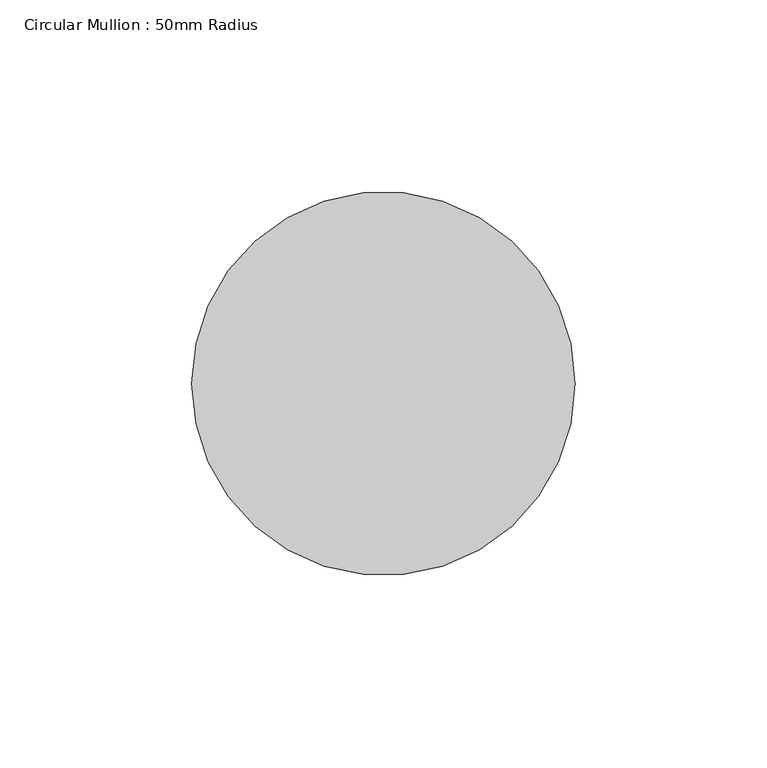
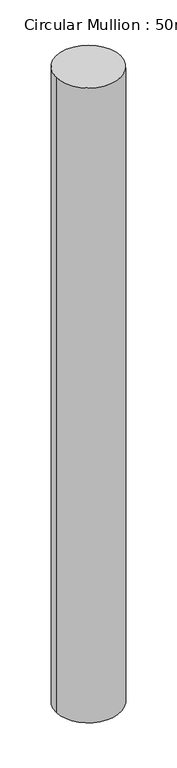
"""IFC4 building model written with IfcOpenShell, lengths in millimetres: member geometry, Circular Mullion : 50mm Radius."""

import ifcopenshell
import ifcopenshell.guid

model = None  # the IFC model being written
_history = None  # IfcOwnerHistory: only IFC2X3 demands one
_inside = {}  # id of a spatial element -> (the spatial element, [elements in it])
_under = {}  # id of a project, library or spatial element -> (it, [spatial elements below it])
_declared = {}  # id of a project -> (the project, [libraries it declares])
_typed = {}  # id of a type object -> (the type object, [elements of that type])
_made_of = {}  # id of a material, layer set ... -> (it, [elements and type objects made of it])


def new_model(schema):
    """Start an empty IFC model of exactly this schema.

    Asked for "IFC4X3", IfcOpenShell would pick the latest addendum, in which some entities
    have other attributes; the version numbers below select the first issue.
    IFC2X3 requires an IfcOwnerHistory on every rooted entity: one is made here for all.
    """
    global model, _history
    if schema == "IFC4X3":
        model = ifcopenshell.file(schema_version=(4, 3, 0, 0))
    else:
        model = ifcopenshell.file(schema=schema)
    _inside.clear()
    _under.clear()
    _declared.clear()
    _typed.clear()
    _made_of.clear()
    _history = None
    if model.schema == "IFC2X3":
        org = make("IfcOrganization", Name="unknown")
        user = make(
            "IfcPersonAndOrganization",
            ThePerson=make("IfcPerson", FamilyName="unknown"),
            TheOrganization=org,
        )
        app = make(
            "IfcApplication",
            ApplicationDeveloper=org,
            Version="unknown",
            ApplicationFullName="unknown",
            ApplicationIdentifier="unknown",
        )
        _history = make(
            "IfcOwnerHistory",
            OwningUser=user,
            OwningApplication=app,
            ChangeAction="ADDED",
            CreationDate=0,
        )
    return model


def make(cls, **values):
    """One entity of the class cls with the attributes given. An attribute that is None is left unset."""
    return model.create_entity(
        cls, **{name: value for name, value in values.items() if value is not None}
    )


def rooted(cls, **values):
    """An entity with a GlobalId (a new one), such as an element, a storey or a relation."""
    return make(cls, GlobalId=ifcopenshell.guid.new(), OwnerHistory=_history, **values)


def si_unit(unit_type, name, prefix=None):
    """IfcSIUnit, for example si_unit("LENGTHUNIT", "METRE", prefix="MILLI")."""
    return make("IfcSIUnit", UnitType=unit_type, Prefix=prefix, Name=name)


def assignment(units):
    """IfcUnitAssignment: the units of a project."""
    return None if units is None else make("IfcUnitAssignment", Units=units)


def point(xyz):
    """IfcCartesianPoint."""
    return None if xyz is None else make("IfcCartesianPoint", Coordinates=xyz)


def direction(xyz):
    """IfcDirection."""
    return None if xyz is None else make("IfcDirection", DirectionRatios=xyz)


def frame(location, z_axis=None, x_axis=None):
    """IfcAxis2Placement3D, a coordinate frame: its origin and axes. An axis left out is left unset."""
    return make(
        "IfcAxis2Placement3D",
        Location=point(location),
        Axis=direction(z_axis),
        RefDirection=direction(x_axis),
    )


def frame_2d(location, x_axis=None):
    """IfcAxis2Placement2D, a coordinate frame in the plane: its origin and x axis."""
    return make(
        "IfcAxis2Placement2D", Location=point(location), RefDirection=direction(x_axis)
    )


def origin():
    """The frame at (0, 0, 0) with its axes left unset."""
    return frame((0.0, 0.0, 0.0))


def origin_2d():
    """The frame at (0, 0) in the plane with its x axis left unset."""
    return frame_2d((0.0, 0.0))


def place(relative_to, where):
    """IfcLocalPlacement: puts the frame where relative to a parent placement (None: the world)."""
    return make(
        "IfcLocalPlacement", PlacementRelTo=relative_to, RelativePlacement=where
    )


def context(
    kind, dimensions, precision=None, world=None, true_north=None, identifier=None
):
    """IfcGeometricRepresentationContext, for example the 3D "Model" context."""
    return make(
        "IfcGeometricRepresentationContext",
        ContextIdentifier=identifier,
        ContextType=kind,
        CoordinateSpaceDimension=dimensions,
        Precision=precision,
        WorldCoordinateSystem=world,
        TrueNorth=true_north,
    )


def project(units=None, contexts=None):
    """IfcProject with its units and contexts."""
    return rooted(
        "IfcProject",
        Name="project",
        RepresentationContexts=contexts,
        UnitsInContext=assignment(units),
    )


def spatial(cls, under=None, at=None, **own):
    """A site, building, storey or space (cls), placed at a placement, below another one or the project."""
    s = rooted(cls, ObjectPlacement=at, **own)
    if under is not None:
        _under.setdefault(under.id(), (under, []))[1].append(s)
    return s


def circle_curve(where, radius):
    """IfcCircle in the frame where."""
    return make("IfcCircle", Position=where, Radius=radius)


def trimmed(basis, trim1, trim2, sense, master):
    """IfcTrimmedCurve: the piece of a basis curve between two trims."""
    return make(
        "IfcTrimmedCurve",
        BasisCurve=basis,
        Trim1=trim1,
        Trim2=trim2,
        SenseAgreement=sense,
        MasterRepresentation=master,
    )


def segment(curve, same_sense, transition):
    """IfcCompositeCurveSegment."""
    return make(
        "IfcCompositeCurveSegment",
        Transition=transition,
        SameSense=same_sense,
        ParentCurve=curve,
    )


def composite_curve(segments, self_intersect=None):
    """IfcCompositeCurve: segments joined end to end."""
    return make("IfcCompositeCurve", Segments=segments, SelfIntersect=self_intersect)


def outline(outer, holes=None, kind="AREA"):
    """IfcArbitraryClosedProfileDef: a profile drawn as a closed curve; with holes, ...WithVoids."""
    if holes is None:
        return make("IfcArbitraryClosedProfileDef", ProfileType=kind, OuterCurve=outer)
    return make(
        "IfcArbitraryProfileDefWithVoids",
        ProfileType=kind,
        OuterCurve=outer,
        InnerCurves=holes,
    )


def extrude(swept, where, along, depth):
    """IfcExtrudedAreaSolid: the profile swept, set in the frame where, extruded along a direction by depth."""
    return make(
        "IfcExtrudedAreaSolid",
        SweptArea=swept,
        Position=where,
        ExtrudedDirection=direction(along),
        Depth=depth,
    )


def shape(context_of_items, identifier, shape_type, items):
    """IfcShapeRepresentation: the items that make up one representation, for example the "Body"."""
    return make(
        "IfcShapeRepresentation",
        ContextOfItems=context_of_items,
        RepresentationIdentifier=identifier,
        RepresentationType=shape_type,
        Items=items,
    )


def source(mapping_origin, context_of_items, identifier, shape_type, items):
    """IfcRepresentationMap: a shape defined once, which mapped items show again and again."""
    return make(
        "IfcRepresentationMap",
        MappingOrigin=mapping_origin,
        MappedRepresentation=shape(context_of_items, identifier, shape_type, items),
    )


def transform(
    local_origin,
    x_axis=None,
    y_axis=None,
    z_axis=None,
    scale=None,
    scale2=None,
    scale3=None,
    uniform=True,
):
    """IfcCartesianTransformationOperator3D, or its non-uniform kind. x_axis, y_axis, z_axis: its Axis1, 2, 3."""
    if uniform:
        return make(
            "IfcCartesianTransformationOperator3D",
            Axis1=direction(x_axis),
            Axis2=direction(y_axis),
            LocalOrigin=point(local_origin),
            Scale=scale,
            Axis3=direction(z_axis),
        )
    return make(
        "IfcCartesianTransformationOperator3DnonUniform",
        Axis1=direction(x_axis),
        Axis2=direction(y_axis),
        LocalOrigin=point(local_origin),
        Scale=scale,
        Axis3=direction(z_axis),
        Scale2=scale2,
        Scale3=scale3,
    )


def mapped(mapping_source, mapping_target):
    """IfcMappedItem: shows the shape of a source again, moved by a transform."""
    return make(
        "IfcMappedItem", MappingSource=mapping_source, MappingTarget=mapping_target
    )


def made_of(thing, what):
    """Note that an element or type object is made of a material, layer set ...; save() writes the relation."""
    if what is not None:
        _made_of.setdefault(what.id(), (what, []))[1].append(thing)
    return thing


def element(
    cls,
    number,
    at=None,
    inside=None,
    cuts=None,
    type_object=None,
    material=None,
    context=None,
    identifier="Body",
    shape_type=None,
    held_by="IfcProductDefinitionShape",
    body=None,
    shapes=None,
    **own,
):
    """One element of the class cls, such as IfcWall. Its Tag is "e" and its number.

    at: its placement. inside: the storey or other place that contains it. cuts: it is an
    opening in that element (IfcRelVoidsElement). A single representation is given by context,
    identifier, shape_type and body (its items); several are given by shapes. held_by: the class
    of the entity that holds the representations. save() writes the other relations.
    """
    e = rooted(cls, Tag="e%d" % number, ObjectPlacement=at, **own)
    if body is not None:
        shapes = [shape(context, identifier, shape_type, body)]
    if shapes is not None:
        e.Representation = make(held_by, Representations=shapes)
    if inside is not None:
        _inside.setdefault(inside.id(), (inside, []))[1].append(e)
    if cuts is not None:
        rooted(
            "IfcRelVoidsElement", RelatingBuildingElement=cuts, RelatedOpeningElement=e
        )
    if type_object is not None:
        _typed.setdefault(type_object.id(), (type_object, []))[1].append(e)
    return made_of(e, material)


def aggregate(whole, parts):
    """IfcRelAggregates: a whole, such as a stair, and the parts it consists of."""
    return rooted("IfcRelAggregates", RelatingObject=whole, RelatedObjects=parts)


def save(model, path):
    """Write the relations noted so far, then the file.

    IfcRelAggregates (storeys below a building ...), IfcRelContainedInSpatialStructure (elements
    in a storey), IfcRelDefinesByType, IfcRelAssociatesMaterial and IfcRelDeclares: one each for
    every whole, place, type object, material and project.
    """
    for whole, parts in _under.values():
        aggregate(whole, parts)
    for where, things in _inside.values():
        rooted(
            "IfcRelContainedInSpatialStructure",
            RelatedElements=things,
            RelatingStructure=where,
        )
    for kind, things in _typed.values():
        rooted("IfcRelDefinesByType", RelatedObjects=things, RelatingType=kind)
    for what, things in _made_of.values():
        rooted("IfcRelAssociatesMaterial", RelatedObjects=things, RelatingMaterial=what)
    for by, libraries in _declared.values():
        rooted("IfcRelDeclares", RelatingContext=by, RelatedDefinitions=libraries)
    model.write(path)


def circular_mullion_50mm_radius_d9d2f8d6(model_context):
    return source(origin(), model_context, "Body", "SweptSolid", [
        extrude(outline(composite_curve([segment(trimmed(circle_curve(origin_2d(), 50.0), [point((50.0, 0.0))], [point((-50.0, 0.0))], False, "CARTESIAN"), True, "CONTINUOUS"), segment(trimmed(circle_curve(origin_2d(), 50.0), [point((-50.0, 0.0))], [point((50.0, 0.0))], False, "CARTESIAN"), True, "CONTINUOUS")], self_intersect=False)), frame((0.0, 0.0, -1037.8609437), z_axis=(0.0, 0.0, 1.0), x_axis=(1.0, 0.0, 0.0)), (0.0, 0.0, 1.0), 1037.8609437),
    ])


if __name__ == "__main__":
    model = new_model("IFC4")
    model_context = context("Model", 3, world=origin())
    ifc_project = project(units=[si_unit("LENGTHUNIT", "METRE", prefix="MILLI")], contexts=[model_context])
    site = spatial("IfcSite", under=ifc_project)
    building = spatial("IfcBuilding", under=site)
    placement = place(None, origin())
    circular_mullion_50mm_radius_shape = circular_mullion_50mm_radius_d9d2f8d6(model_context)
    element("IfcMember", 1, ObjectType="Circular Mullion : 50mm Radius", at=placement, inside=building, context=model_context, shape_type="MappedRepresentation", body=[
        mapped(circular_mullion_50mm_radius_shape, transform((0.0, 0.0, 0.0), x_axis=(1.0, 0.0, 0.0), y_axis=(0.0, 1.0, 0.0), z_axis=(0.0, 0.0, 1.0))),
    ])
    save(model, "model.ifc")

# Revit data of these elements
# Type "Circular Mullion : 50mm Radius"
#   built-in parameter 1007350 = 0.164042 (stored number, unit not read)
# Element 1 (IfcMember, "Circular Mullion : 50mm Radius")
#   Materials on its faces: "Aluminium"
# Materials
#   "Aluminium": class "Metal", colour RGB 247 247 247, transparency 0, Description = "Aluminium 6061", Cost = 0
